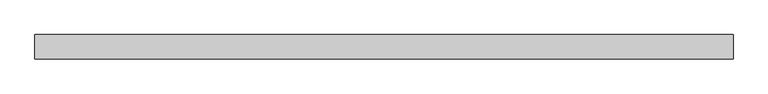
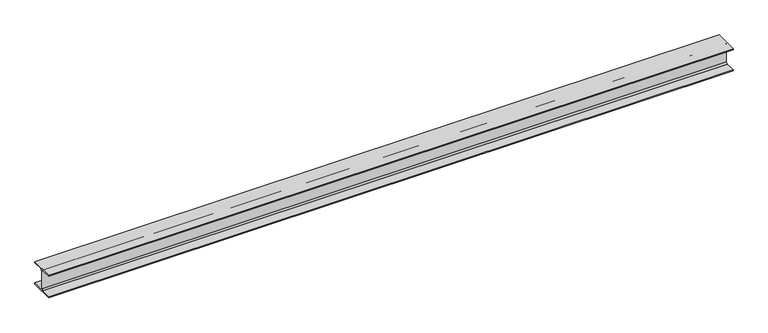
"""IFC4 building model written with IfcOpenShell, lengths in millimetres: beam geometry, 0912_Steel Framing_H-KSD3502 : H_SB_ASB_H-300x300x10x15."""

import ifcopenshell
import ifcopenshell.guid

model = None  # the IFC model being written
_history = None  # IfcOwnerHistory: only IFC2X3 demands one
_inside = {}  # id of a spatial element -> (the spatial element, [elements in it])
_under = {}  # id of a project, library or spatial element -> (it, [spatial elements below it])
_declared = {}  # id of a project -> (the project, [libraries it declares])
_typed = {}  # id of a type object -> (the type object, [elements of that type])
_made_of = {}  # id of a material, layer set ... -> (it, [elements and type objects made of it])


def new_model(schema):
    """Start an empty IFC model of exactly this schema.

    Asked for "IFC4X3", IfcOpenShell would pick the latest addendum, in which some entities
    have other attributes; the version numbers below select the first issue.
    IFC2X3 requires an IfcOwnerHistory on every rooted entity: one is made here for all.
    """
    global model, _history
    if schema == "IFC4X3":
        model = ifcopenshell.file(schema_version=(4, 3, 0, 0))
    else:
        model = ifcopenshell.file(schema=schema)
    _inside.clear()
    _under.clear()
    _declared.clear()
    _typed.clear()
    _made_of.clear()
    _history = None
    if model.schema == "IFC2X3":
        org = make("IfcOrganization", Name="unknown")
        user = make(
            "IfcPersonAndOrganization",
            ThePerson=make("IfcPerson", FamilyName="unknown"),
            TheOrganization=org,
        )
        app = make(
            "IfcApplication",
            ApplicationDeveloper=org,
            Version="unknown",
            ApplicationFullName="unknown",
            ApplicationIdentifier="unknown",
        )
        _history = make(
            "IfcOwnerHistory",
            OwningUser=user,
            OwningApplication=app,
            ChangeAction="ADDED",
            CreationDate=0,
        )
    return model


def make(cls, **values):
    """One entity of the class cls with the attributes given. An attribute that is None is left unset."""
    return model.create_entity(
        cls, **{name: value for name, value in values.items() if value is not None}
    )


def rooted(cls, **values):
    """An entity with a GlobalId (a new one), such as an element, a storey or a relation."""
    return make(cls, GlobalId=ifcopenshell.guid.new(), OwnerHistory=_history, **values)


def si_unit(unit_type, name, prefix=None):
    """IfcSIUnit, for example si_unit("LENGTHUNIT", "METRE", prefix="MILLI")."""
    return make("IfcSIUnit", UnitType=unit_type, Prefix=prefix, Name=name)


def assignment(units):
    """IfcUnitAssignment: the units of a project."""
    return None if units is None else make("IfcUnitAssignment", Units=units)


def point(xyz):
    """IfcCartesianPoint."""
    return None if xyz is None else make("IfcCartesianPoint", Coordinates=xyz)


def direction(xyz):
    """IfcDirection."""
    return None if xyz is None else make("IfcDirection", DirectionRatios=xyz)


def frame(location, z_axis=None, x_axis=None):
    """IfcAxis2Placement3D, a coordinate frame: its origin and axes. An axis left out is left unset."""
    return make(
        "IfcAxis2Placement3D",
        Location=point(location),
        Axis=direction(z_axis),
        RefDirection=direction(x_axis),
    )


def frame_2d(location, x_axis=None):
    """IfcAxis2Placement2D, a coordinate frame in the plane: its origin and x axis."""
    return make(
        "IfcAxis2Placement2D", Location=point(location), RefDirection=direction(x_axis)
    )


def origin():
    """The frame at (0, 0, 0) with its axes left unset."""
    return frame((0.0, 0.0, 0.0))


def place(relative_to, where):
    """IfcLocalPlacement: puts the frame where relative to a parent placement (None: the world)."""
    return make(
        "IfcLocalPlacement", PlacementRelTo=relative_to, RelativePlacement=where
    )


def context(
    kind, dimensions, precision=None, world=None, true_north=None, identifier=None
):
    """IfcGeometricRepresentationContext, for example the 3D "Model" context."""
    return make(
        "IfcGeometricRepresentationContext",
        ContextIdentifier=identifier,
        ContextType=kind,
        CoordinateSpaceDimension=dimensions,
        Precision=precision,
        WorldCoordinateSystem=world,
        TrueNorth=true_north,
    )


def project(units=None, contexts=None):
    """IfcProject with its units and contexts."""
    return rooted(
        "IfcProject",
        Name="project",
        RepresentationContexts=contexts,
        UnitsInContext=assignment(units),
    )


def spatial(cls, under=None, at=None, **own):
    """A site, building, storey or space (cls), placed at a placement, below another one or the project."""
    s = rooted(cls, ObjectPlacement=at, **own)
    if under is not None:
        _under.setdefault(under.id(), (under, []))[1].append(s)
    return s


def polyline(points):
    """IfcPolyline through the points."""
    return make("IfcPolyline", Points=[point(p) for p in points])


def circle_curve(where, radius):
    """IfcCircle in the frame where."""
    return make("IfcCircle", Position=where, Radius=radius)


def trimmed(basis, trim1, trim2, sense, master):
    """IfcTrimmedCurve: the piece of a basis curve between two trims."""
    return make(
        "IfcTrimmedCurve",
        BasisCurve=basis,
        Trim1=trim1,
        Trim2=trim2,
        SenseAgreement=sense,
        MasterRepresentation=master,
    )


def segment(curve, same_sense, transition):
    """IfcCompositeCurveSegment."""
    return make(
        "IfcCompositeCurveSegment",
        Transition=transition,
        SameSense=same_sense,
        ParentCurve=curve,
    )


def composite_curve(segments, self_intersect=None):
    """IfcCompositeCurve: segments joined end to end."""
    return make("IfcCompositeCurve", Segments=segments, SelfIntersect=self_intersect)


def outline(outer, holes=None, kind="AREA"):
    """IfcArbitraryClosedProfileDef: a profile drawn as a closed curve; with holes, ...WithVoids."""
    if holes is None:
        return make("IfcArbitraryClosedProfileDef", ProfileType=kind, OuterCurve=outer)
    return make(
        "IfcArbitraryProfileDefWithVoids",
        ProfileType=kind,
        OuterCurve=outer,
        InnerCurves=holes,
    )


def extrude(swept, where, along, depth):
    """IfcExtrudedAreaSolid: the profile swept, set in the frame where, extruded along a direction by depth."""
    return make(
        "IfcExtrudedAreaSolid",
        SweptArea=swept,
        Position=where,
        ExtrudedDirection=direction(along),
        Depth=depth,
    )


def shape(context_of_items, identifier, shape_type, items):
    """IfcShapeRepresentation: the items that make up one representation, for example the "Body"."""
    return make(
        "IfcShapeRepresentation",
        ContextOfItems=context_of_items,
        RepresentationIdentifier=identifier,
        RepresentationType=shape_type,
        Items=items,
    )


def source(mapping_origin, context_of_items, identifier, shape_type, items):
    """IfcRepresentationMap: a shape defined once, which mapped items show again and again."""
    return make(
        "IfcRepresentationMap",
        MappingOrigin=mapping_origin,
        MappedRepresentation=shape(context_of_items, identifier, shape_type, items),
    )


def transform(
    local_origin,
    x_axis=None,
    y_axis=None,
    z_axis=None,
    scale=None,
    scale2=None,
    scale3=None,
    uniform=True,
):
    """IfcCartesianTransformationOperator3D, or its non-uniform kind. x_axis, y_axis, z_axis: its Axis1, 2, 3."""
    if uniform:
        return make(
            "IfcCartesianTransformationOperator3D",
            Axis1=direction(x_axis),
            Axis2=direction(y_axis),
            LocalOrigin=point(local_origin),
            Scale=scale,
            Axis3=direction(z_axis),
        )
    return make(
        "IfcCartesianTransformationOperator3DnonUniform",
        Axis1=direction(x_axis),
        Axis2=direction(y_axis),
        LocalOrigin=point(local_origin),
        Scale=scale,
        Axis3=direction(z_axis),
        Scale2=scale2,
        Scale3=scale3,
    )


def mapped(mapping_source, mapping_target):
    """IfcMappedItem: shows the shape of a source again, moved by a transform."""
    return make(
        "IfcMappedItem", MappingSource=mapping_source, MappingTarget=mapping_target
    )


def made_of(thing, what):
    """Note that an element or type object is made of a material, layer set ...; save() writes the relation."""
    if what is not None:
        _made_of.setdefault(what.id(), (what, []))[1].append(thing)
    return thing


def element(
    cls,
    number,
    at=None,
    inside=None,
    cuts=None,
    type_object=None,
    material=None,
    context=None,
    identifier="Body",
    shape_type=None,
    held_by="IfcProductDefinitionShape",
    body=None,
    shapes=None,
    **own,
):
    """One element of the class cls, such as IfcWall. Its Tag is "e" and its number.

    at: its placement. inside: the storey or other place that contains it. cuts: it is an
    opening in that element (IfcRelVoidsElement). A single representation is given by context,
    identifier, shape_type and body (its items); several are given by shapes. held_by: the class
    of the entity that holds the representations. save() writes the other relations.
    """
    e = rooted(cls, Tag="e%d" % number, ObjectPlacement=at, **own)
    if body is not None:
        shapes = [shape(context, identifier, shape_type, body)]
    if shapes is not None:
        e.Representation = make(held_by, Representations=shapes)
    if inside is not None:
        _inside.setdefault(inside.id(), (inside, []))[1].append(e)
    if cuts is not None:
        rooted(
            "IfcRelVoidsElement", RelatingBuildingElement=cuts, RelatedOpeningElement=e
        )
    if type_object is not None:
        _typed.setdefault(type_object.id(), (type_object, []))[1].append(e)
    return made_of(e, material)


def aggregate(whole, parts):
    """IfcRelAggregates: a whole, such as a stair, and the parts it consists of."""
    return rooted("IfcRelAggregates", RelatingObject=whole, RelatedObjects=parts)


def save(model, path):
    """Write the relations noted so far, then the file.

    IfcRelAggregates (storeys below a building ...), IfcRelContainedInSpatialStructure (elements
    in a storey), IfcRelDefinesByType, IfcRelAssociatesMaterial and IfcRelDeclares: one each for
    every whole, place, type object, material and project.
    """
    for whole, parts in _under.values():
        aggregate(whole, parts)
    for where, things in _inside.values():
        rooted(
            "IfcRelContainedInSpatialStructure",
            RelatedElements=things,
            RelatingStructure=where,
        )
    for kind, things in _typed.values():
        rooted("IfcRelDefinesByType", RelatedObjects=things, RelatingType=kind)
    for what, things in _made_of.values():
        rooted("IfcRelAssociatesMaterial", RelatedObjects=things, RelatingMaterial=what)
    for by, libraries in _declared.values():
        rooted("IfcRelDeclares", RelatingContext=by, RelatedDefinitions=libraries)
    model.write(path)


def beam_276f2b7d(model_context):
    return source(origin(), model_context, "Body", "SweptSolid", [
        extrude(outline(composite_curve([segment(polyline([(150.0, -135.0), (150.0, -150.0), (-150.0, -150.0), (-150.0, -135.0), (-23.0, -135.0)]), True, "CONTINUOUS"), segment(trimmed(circle_curve(frame_2d((-23.0, -117.0)), 18.0), [point((-23.0, -135.0))], [point((-5.0, -117.0))], True, "CARTESIAN"), True, "CONTINUOUS"), segment(polyline([(-5.0, -117.0), (-5.0, 117.0)]), True, "CONTINUOUS"), segment(trimmed(circle_curve(frame_2d((-23.0, 117.0)), 18.0), [point((-5.0, 117.0))], [point((-23.0, 135.0))], True, "CARTESIAN"), True, "CONTINUOUS"), segment(polyline([(-23.0, 135.0), (-150.0, 135.0), (-150.0, 150.0), (150.0, 150.0), (150.0, 135.0), (23.0, 135.0)]), True, "CONTINUOUS"), segment(trimmed(circle_curve(frame_2d((23.0, 117.0)), 18.0), [point((23.0, 135.0))], [point((5.0, 117.0))], True, "CARTESIAN"), True, "CONTINUOUS"), segment(polyline([(5.0, 117.0), (5.0, -117.0)]), True, "CONTINUOUS"), segment(trimmed(circle_curve(frame_2d((23.0, -117.0)), 18.0), [point((5.0, -117.0))], [point((23.0, -135.0))], True, "CARTESIAN"), True, "CONTINUOUS"), segment(polyline([(23.0, -135.0), (150.0, -135.0)]), True, "CONTINUOUS")], self_intersect=False)), frame((-4272.9251782, 0.0, 0.0), z_axis=(1.0, 0.0, 0.0), x_axis=(0.0, 1.0, 0.0)), (0.0, 0.0, 1.0), 8647.1704515),
    ])


if __name__ == "__main__":
    model = new_model("IFC4")
    model_context = context("Model", 3, world=origin())
    ifc_project = project(units=[si_unit("LENGTHUNIT", "METRE", prefix="MILLI")], contexts=[model_context])
    site = spatial("IfcSite", under=ifc_project)
    building = spatial("IfcBuilding", under=site)
    placement = place(None, origin())
    beam_shape = beam_276f2b7d(model_context)
    element("IfcBeam", 1, ObjectType="0912_Steel Framing_H-KSD3502 : H_SB_ASB_H-300x300x10x15", at=placement, inside=building, context=model_context, shape_type="MappedRepresentation", body=[
        mapped(beam_shape, transform((0.0, 0.0, 0.0), x_axis=(1.0, 0.0, 0.0), y_axis=(0.0, 1.0, 0.0), z_axis=(0.0, 0.0, 1.0))),
    ])
    save(model, "model.ifc")

# Revit data of these elements
# Type "0912_Steel Framing_H-KSD3502 : H_SB_ASB_H-300x300x10x15"
#   H_WM Code_1 = "S01AA001-00001 | Main Steel Structure Fabrication Work | Shelter/Building | Heavy Steel - Standard (Weight≥90KG/M) | Material: (   )"
#   H_WM Code_2 = "S03AA027-00001 | Main Steel Structure Erection Work | Shelter/Building | Heavy Steel (Weight≥90KG/M) | Material: (   )"
#   H_WM Code_3 = "S01AA010-00001 | Main Steel Structure Fabrication Work | Shelter/Building | Steel Painting/Coating | for Non-Fireproofed Steel Surface, Surface Preparation, Primer, Second & Final Coat | Material: (   )"
#   H_Q'ty Cal Type Tag = "SB-Q2"
#   Width = 30.0 cm
#   Web Thickness = 1.0 cm
#   Web Fillet = 1.8 cm
#   Warping Constant = 1370000.0 cm⁶
#   W = 0
#   Torsional Moment of Inertia = 77.00 cm⁴
#   Section Area = 119.8 cm²
#   Plastic Modulus weak axis = 684.0 cm³
#   Plastic Modulus strong axis = 1500.0 cm³
#   Perimeter = 1.75 m²/m
#   Nominal Weight = 94.00 kgf/m
#   Moment of Inertia weak axis = 6750.00 cm⁴
#   Moment of Inertia strong axis = 20400.00 cm⁴
#   Height = 30.0 cm
#   Flange Thickness = 1.5 cm
#   Elastic Modulus weak axis = 450.0 cm³
#   Elastic Modulus strong axis = 1360.0 cm³
#   Centroid Vertical = 15.0 cm
#   Centroid Horizontal = 15.0 cm
#   Ix = 204000000
#   Length [instance default] = 1.5240 m
#   Zx = 1500000
#   b = 0.3000 m
#   h = 0.3000 m
#   r = 0.0180 m
#   s = 0.0100 m
#   t = 0.0150 m
#   A = 0.01198 m²
#   Structural Material [instance default] = Steel, 45-345
#   Assembly Code = ""
# Element 1 (IfcBeam, "0912_Steel Framing_H-KSD3502 : H_SB_ASB_H-300x300x10x15")
#   Structural Material = none
# Materials
#   "Steel, 45-345": class "Metal", colour RGB 189 187 185, transparency 0, Description = "Steel 345 MPa", Cost = 0
